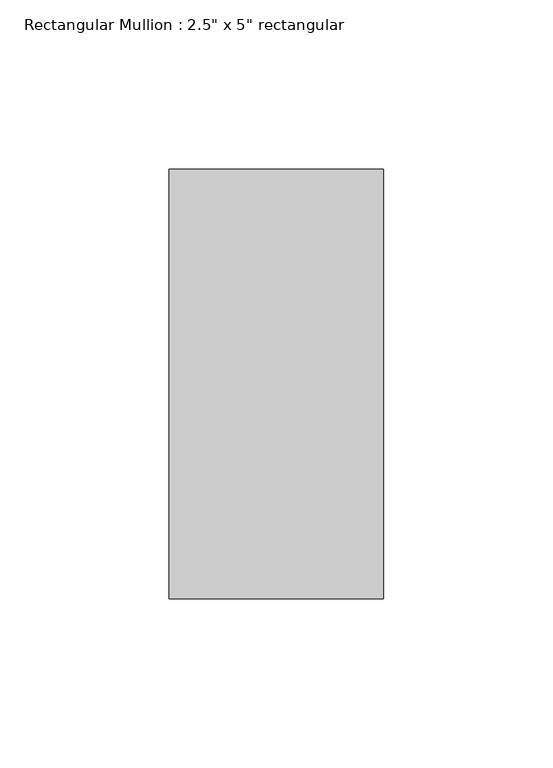
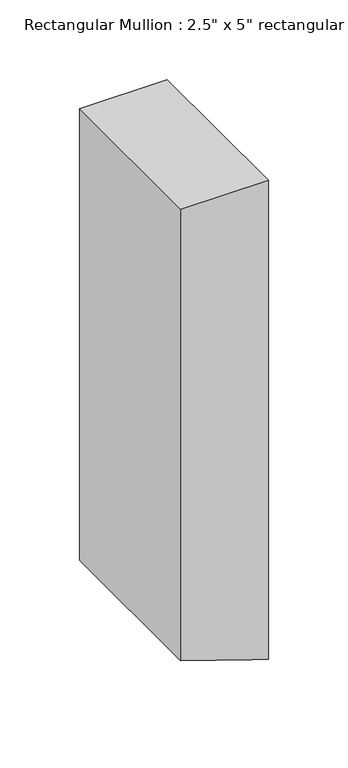
"""IFC4 building model written with IfcOpenShell, lengths in millimetres: member geometry."""

from ifc_helpers import new_model, si_unit, frame, origin, place, context, project, spatial, polyline, outline, extrude, source, transform, mapped, element, save


def member_056e3271(model_context):
    return source(origin(), model_context, "Body", "SweptSolid", [
        extrude(outline(polyline([(0.0, 31.75), (0.0, -31.75), (-345.8151229, -31.75), (-363.0919439, 20.0804631), (-366.9817895, 31.75), (0.0, 31.75)])), frame((0.0, -63.5, 0.0), z_axis=(0.0, 1.0, 0.0), x_axis=(0.0, 0.0, 1.0)), (0.0, 0.0, 1.0), 127.0),
    ])


if __name__ == "__main__":
    model = new_model("IFC4")
    model_context = context("Model", 3, world=origin())
    ifc_project = project(units=[si_unit("LENGTHUNIT", "METRE", prefix="MILLI")], contexts=[model_context])
    site = spatial("IfcSite", under=ifc_project)
    building = spatial("IfcBuilding", under=site)
    placement = place(None, origin())
    member_shape = member_056e3271(model_context)
    element("IfcMember", 1, ObjectType="Rectangular Mullion : 2.5\" x 5\" rectangular", at=placement, inside=building, context=model_context, shape_type="MappedRepresentation", body=[
        mapped(member_shape, transform((0.0, 0.0, 0.0), x_axis=(1.0, 0.0, 0.0), y_axis=(0.0, 1.0, 0.0), z_axis=(0.0, 0.0, 1.0))),
    ])
    save(model, "model.ifc")

# Revit data of these elements
# Type "Rectangular Mullion : 2.5\" x 5\" rectangular"
#   built-in parameter 1007304 = 0.416667 (stored number, unit not read)
#   built-in parameter 1007301 = 0.104167 (stored number, unit not read)
#   built-in parameter 1007300 = 0.104167 (stored number, unit not read)
# Element 1 (IfcMember, "Rectangular Mullion : 2.5\" x 5\" rectangular")
#   Materials on its faces: "Metal - Aluminum"
# Materials
#   "Metal - Aluminum": class "Metal", colour RGB 140 140 140, transparency 0
